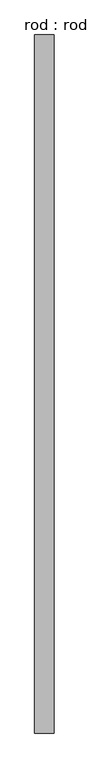
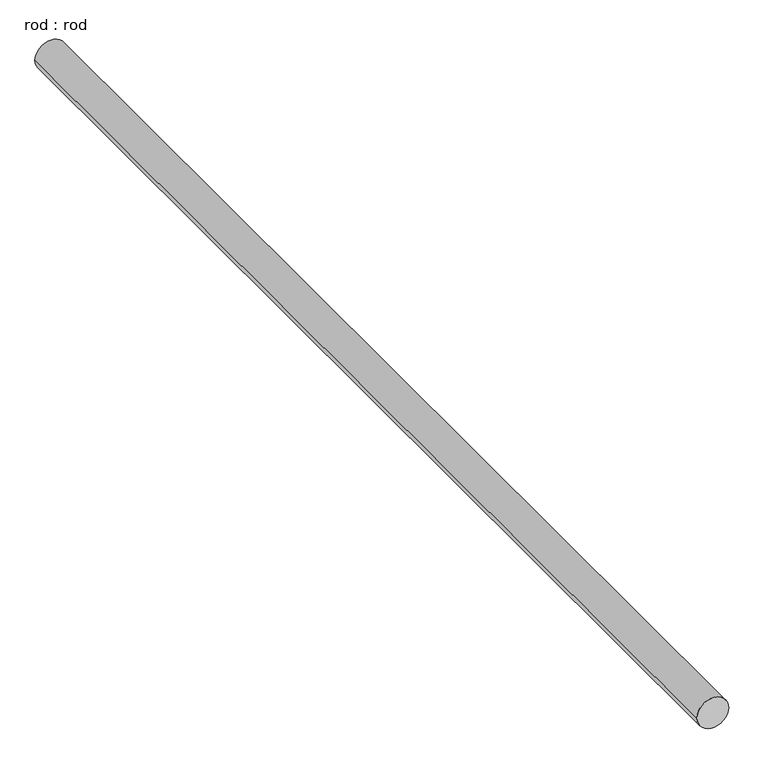
"""IFC4 building model written with IfcOpenShell, lengths in millimetres: proxy geometry, rod : rod."""

import ifcopenshell
import ifcopenshell.guid

model = None  # the IFC model being written
_history = None  # IfcOwnerHistory: only IFC2X3 demands one
_inside = {}  # id of a spatial element -> (the spatial element, [elements in it])
_under = {}  # id of a project, library or spatial element -> (it, [spatial elements below it])
_declared = {}  # id of a project -> (the project, [libraries it declares])
_typed = {}  # id of a type object -> (the type object, [elements of that type])
_made_of = {}  # id of a material, layer set ... -> (it, [elements and type objects made of it])


def new_model(schema):
    """Start an empty IFC model of exactly this schema.

    Asked for "IFC4X3", IfcOpenShell would pick the latest addendum, in which some entities
    have other attributes; the version numbers below select the first issue.
    IFC2X3 requires an IfcOwnerHistory on every rooted entity: one is made here for all.
    """
    global model, _history
    if schema == "IFC4X3":
        model = ifcopenshell.file(schema_version=(4, 3, 0, 0))
    else:
        model = ifcopenshell.file(schema=schema)
    _inside.clear()
    _under.clear()
    _declared.clear()
    _typed.clear()
    _made_of.clear()
    _history = None
    if model.schema == "IFC2X3":
        org = make("IfcOrganization", Name="unknown")
        user = make(
            "IfcPersonAndOrganization",
            ThePerson=make("IfcPerson", FamilyName="unknown"),
            TheOrganization=org,
        )
        app = make(
            "IfcApplication",
            ApplicationDeveloper=org,
            Version="unknown",
            ApplicationFullName="unknown",
            ApplicationIdentifier="unknown",
        )
        _history = make(
            "IfcOwnerHistory",
            OwningUser=user,
            OwningApplication=app,
            ChangeAction="ADDED",
            CreationDate=0,
        )
    return model


def make(cls, **values):
    """One entity of the class cls with the attributes given. An attribute that is None is left unset."""
    return model.create_entity(
        cls, **{name: value for name, value in values.items() if value is not None}
    )


def rooted(cls, **values):
    """An entity with a GlobalId (a new one), such as an element, a storey or a relation."""
    return make(cls, GlobalId=ifcopenshell.guid.new(), OwnerHistory=_history, **values)


def si_unit(unit_type, name, prefix=None):
    """IfcSIUnit, for example si_unit("LENGTHUNIT", "METRE", prefix="MILLI")."""
    return make("IfcSIUnit", UnitType=unit_type, Prefix=prefix, Name=name)


def assignment(units):
    """IfcUnitAssignment: the units of a project."""
    return None if units is None else make("IfcUnitAssignment", Units=units)


def point(xyz):
    """IfcCartesianPoint."""
    return None if xyz is None else make("IfcCartesianPoint", Coordinates=xyz)


def direction(xyz):
    """IfcDirection."""
    return None if xyz is None else make("IfcDirection", DirectionRatios=xyz)


def frame(location, z_axis=None, x_axis=None):
    """IfcAxis2Placement3D, a coordinate frame: its origin and axes. An axis left out is left unset."""
    return make(
        "IfcAxis2Placement3D",
        Location=point(location),
        Axis=direction(z_axis),
        RefDirection=direction(x_axis),
    )


def frame_2d(location, x_axis=None):
    """IfcAxis2Placement2D, a coordinate frame in the plane: its origin and x axis."""
    return make(
        "IfcAxis2Placement2D", Location=point(location), RefDirection=direction(x_axis)
    )


def origin():
    """The frame at (0, 0, 0) with its axes left unset."""
    return frame((0.0, 0.0, 0.0))


def place(relative_to, where):
    """IfcLocalPlacement: puts the frame where relative to a parent placement (None: the world)."""
    return make(
        "IfcLocalPlacement", PlacementRelTo=relative_to, RelativePlacement=where
    )


def context(
    kind, dimensions, precision=None, world=None, true_north=None, identifier=None
):
    """IfcGeometricRepresentationContext, for example the 3D "Model" context."""
    return make(
        "IfcGeometricRepresentationContext",
        ContextIdentifier=identifier,
        ContextType=kind,
        CoordinateSpaceDimension=dimensions,
        Precision=precision,
        WorldCoordinateSystem=world,
        TrueNorth=true_north,
    )


def project(units=None, contexts=None):
    """IfcProject with its units and contexts."""
    return rooted(
        "IfcProject",
        Name="project",
        RepresentationContexts=contexts,
        UnitsInContext=assignment(units),
    )


def spatial(cls, under=None, at=None, **own):
    """A site, building, storey or space (cls), placed at a placement, below another one or the project."""
    s = rooted(cls, ObjectPlacement=at, **own)
    if under is not None:
        _under.setdefault(under.id(), (under, []))[1].append(s)
    return s


def circle_curve(where, radius):
    """IfcCircle in the frame where."""
    return make("IfcCircle", Position=where, Radius=radius)


def trimmed(basis, trim1, trim2, sense, master):
    """IfcTrimmedCurve: the piece of a basis curve between two trims."""
    return make(
        "IfcTrimmedCurve",
        BasisCurve=basis,
        Trim1=trim1,
        Trim2=trim2,
        SenseAgreement=sense,
        MasterRepresentation=master,
    )


def segment(curve, same_sense, transition):
    """IfcCompositeCurveSegment."""
    return make(
        "IfcCompositeCurveSegment",
        Transition=transition,
        SameSense=same_sense,
        ParentCurve=curve,
    )


def composite_curve(segments, self_intersect=None):
    """IfcCompositeCurve: segments joined end to end."""
    return make("IfcCompositeCurve", Segments=segments, SelfIntersect=self_intersect)


def outline(outer, holes=None, kind="AREA"):
    """IfcArbitraryClosedProfileDef: a profile drawn as a closed curve; with holes, ...WithVoids."""
    if holes is None:
        return make("IfcArbitraryClosedProfileDef", ProfileType=kind, OuterCurve=outer)
    return make(
        "IfcArbitraryProfileDefWithVoids",
        ProfileType=kind,
        OuterCurve=outer,
        InnerCurves=holes,
    )


def extrude(swept, where, along, depth):
    """IfcExtrudedAreaSolid: the profile swept, set in the frame where, extruded along a direction by depth."""
    return make(
        "IfcExtrudedAreaSolid",
        SweptArea=swept,
        Position=where,
        ExtrudedDirection=direction(along),
        Depth=depth,
    )


def shape(context_of_items, identifier, shape_type, items):
    """IfcShapeRepresentation: the items that make up one representation, for example the "Body"."""
    return make(
        "IfcShapeRepresentation",
        ContextOfItems=context_of_items,
        RepresentationIdentifier=identifier,
        RepresentationType=shape_type,
        Items=items,
    )


def source(mapping_origin, context_of_items, identifier, shape_type, items):
    """IfcRepresentationMap: a shape defined once, which mapped items show again and again."""
    return make(
        "IfcRepresentationMap",
        MappingOrigin=mapping_origin,
        MappedRepresentation=shape(context_of_items, identifier, shape_type, items),
    )


def transform(
    local_origin,
    x_axis=None,
    y_axis=None,
    z_axis=None,
    scale=None,
    scale2=None,
    scale3=None,
    uniform=True,
):
    """IfcCartesianTransformationOperator3D, or its non-uniform kind. x_axis, y_axis, z_axis: its Axis1, 2, 3."""
    if uniform:
        return make(
            "IfcCartesianTransformationOperator3D",
            Axis1=direction(x_axis),
            Axis2=direction(y_axis),
            LocalOrigin=point(local_origin),
            Scale=scale,
            Axis3=direction(z_axis),
        )
    return make(
        "IfcCartesianTransformationOperator3DnonUniform",
        Axis1=direction(x_axis),
        Axis2=direction(y_axis),
        LocalOrigin=point(local_origin),
        Scale=scale,
        Axis3=direction(z_axis),
        Scale2=scale2,
        Scale3=scale3,
    )


def mapped(mapping_source, mapping_target):
    """IfcMappedItem: shows the shape of a source again, moved by a transform."""
    return make(
        "IfcMappedItem", MappingSource=mapping_source, MappingTarget=mapping_target
    )


def made_of(thing, what):
    """Note that an element or type object is made of a material, layer set ...; save() writes the relation."""
    if what is not None:
        _made_of.setdefault(what.id(), (what, []))[1].append(thing)
    return thing


def element(
    cls,
    number,
    at=None,
    inside=None,
    cuts=None,
    type_object=None,
    material=None,
    context=None,
    identifier="Body",
    shape_type=None,
    held_by="IfcProductDefinitionShape",
    body=None,
    shapes=None,
    **own,
):
    """One element of the class cls, such as IfcWall. Its Tag is "e" and its number.

    at: its placement. inside: the storey or other place that contains it. cuts: it is an
    opening in that element (IfcRelVoidsElement). A single representation is given by context,
    identifier, shape_type and body (its items); several are given by shapes. held_by: the class
    of the entity that holds the representations. save() writes the other relations.
    """
    e = rooted(cls, Tag="e%d" % number, ObjectPlacement=at, **own)
    if body is not None:
        shapes = [shape(context, identifier, shape_type, body)]
    if shapes is not None:
        e.Representation = make(held_by, Representations=shapes)
    if inside is not None:
        _inside.setdefault(inside.id(), (inside, []))[1].append(e)
    if cuts is not None:
        rooted(
            "IfcRelVoidsElement", RelatingBuildingElement=cuts, RelatedOpeningElement=e
        )
    if type_object is not None:
        _typed.setdefault(type_object.id(), (type_object, []))[1].append(e)
    return made_of(e, material)


def aggregate(whole, parts):
    """IfcRelAggregates: a whole, such as a stair, and the parts it consists of."""
    return rooted("IfcRelAggregates", RelatingObject=whole, RelatedObjects=parts)


def save(model, path):
    """Write the relations noted so far, then the file.

    IfcRelAggregates (storeys below a building ...), IfcRelContainedInSpatialStructure (elements
    in a storey), IfcRelDefinesByType, IfcRelAssociatesMaterial and IfcRelDeclares: one each for
    every whole, place, type object, material and project.
    """
    for whole, parts in _under.values():
        aggregate(whole, parts)
    for where, things in _inside.values():
        rooted(
            "IfcRelContainedInSpatialStructure",
            RelatedElements=things,
            RelatingStructure=where,
        )
    for kind, things in _typed.values():
        rooted("IfcRelDefinesByType", RelatedObjects=things, RelatingType=kind)
    for what, things in _made_of.values():
        rooted("IfcRelAssociatesMaterial", RelatedObjects=things, RelatingMaterial=what)
    for by, libraries in _declared.values():
        rooted("IfcRelDeclares", RelatingContext=by, RelatedDefinitions=libraries)
    model.write(path)


def rod_rod_bead025f(model_context):
    return source(origin(), model_context, "Body", "SweptSolid", [
        extrude(outline(composite_curve([segment(trimmed(circle_curve(frame_2d((0.0108462, 0.0)), 200.0), [point((0.0108462, 200.0))], [point((0.0108462, -200.0))], False, "CARTESIAN"), True, "CONTINUOUS"), segment(trimmed(circle_curve(frame_2d((0.0108462, 0.0)), 200.0), [point((0.0108462, -200.0))], [point((0.0108462, 200.0))], False, "CARTESIAN"), True, "CONTINUOUS")], self_intersect=False)), frame((0.0, -3126.0213847, 0.0), z_axis=(0.0, 1.0, 0.0), x_axis=(0.0, 0.0, 1.0)), (0.0, 0.0, 1.0), 14437.5),
    ])


if __name__ == "__main__":
    model = new_model("IFC4")
    model_context = context("Model", 3, world=origin())
    ifc_project = project(units=[si_unit("LENGTHUNIT", "METRE", prefix="MILLI")], contexts=[model_context])
    site = spatial("IfcSite", under=ifc_project)
    building = spatial("IfcBuilding", under=site)
    placement = place(None, origin())
    rod_rod_shape = rod_rod_bead025f(model_context)
    element("IfcBuildingElementProxy", 1, Name="rod : rod", ObjectType="rod : rod", at=placement, inside=building, context=model_context, shape_type="MappedRepresentation", body=[
        mapped(rod_rod_shape, transform((0.0, 0.0, 0.0), x_axis=(1.0, 0.0, 0.0), y_axis=(0.0, 1.0, 0.0), z_axis=(0.0, 0.0, 1.0))),
    ])
    save(model, "model.ifc")

# Revit data of these elements
# Type "rod : rod"
#   Default Elevation = 0
